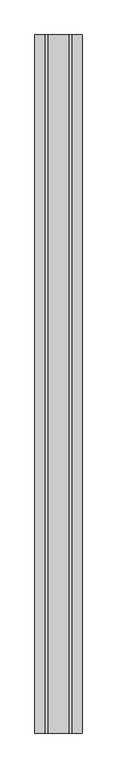
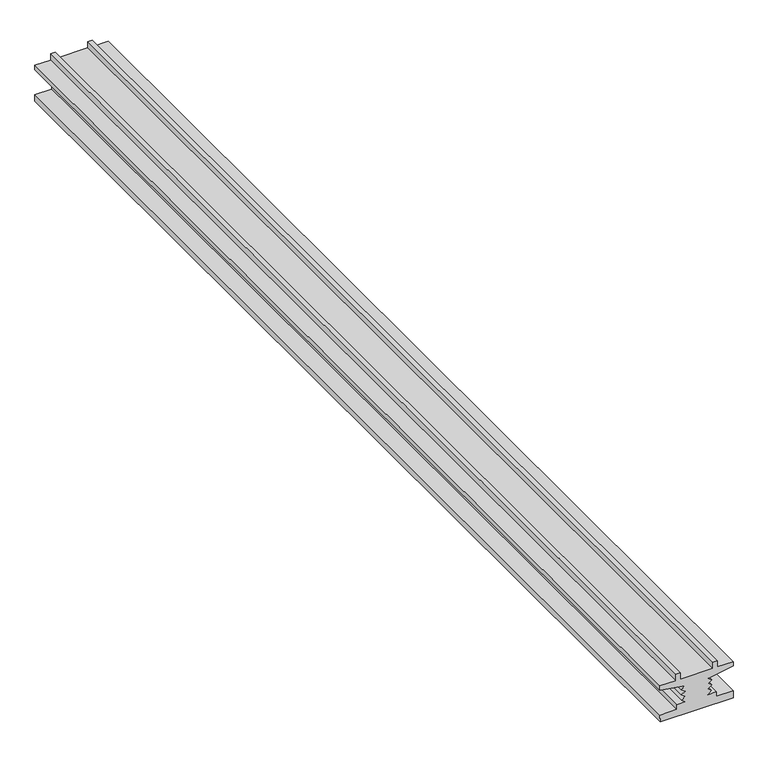
"""IFC4 building model written with IfcOpenShell, lengths in millimetres: proxy geometry, Bison pedestal001 : Bison pedestal001."""

import ifcopenshell
import ifcopenshell.guid

model = None  # the IFC model being written
_history = None  # IfcOwnerHistory: only IFC2X3 demands one
_inside = {}  # id of a spatial element -> (the spatial element, [elements in it])
_under = {}  # id of a project, library or spatial element -> (it, [spatial elements below it])
_declared = {}  # id of a project -> (the project, [libraries it declares])
_typed = {}  # id of a type object -> (the type object, [elements of that type])
_made_of = {}  # id of a material, layer set ... -> (it, [elements and type objects made of it])


def new_model(schema):
    """Start an empty IFC model of exactly this schema.

    Asked for "IFC4X3", IfcOpenShell would pick the latest addendum, in which some entities
    have other attributes; the version numbers below select the first issue.
    IFC2X3 requires an IfcOwnerHistory on every rooted entity: one is made here for all.
    """
    global model, _history
    if schema == "IFC4X3":
        model = ifcopenshell.file(schema_version=(4, 3, 0, 0))
    else:
        model = ifcopenshell.file(schema=schema)
    _inside.clear()
    _under.clear()
    _declared.clear()
    _typed.clear()
    _made_of.clear()
    _history = None
    if model.schema == "IFC2X3":
        org = make("IfcOrganization", Name="unknown")
        user = make(
            "IfcPersonAndOrganization",
            ThePerson=make("IfcPerson", FamilyName="unknown"),
            TheOrganization=org,
        )
        app = make(
            "IfcApplication",
            ApplicationDeveloper=org,
            Version="unknown",
            ApplicationFullName="unknown",
            ApplicationIdentifier="unknown",
        )
        _history = make(
            "IfcOwnerHistory",
            OwningUser=user,
            OwningApplication=app,
            ChangeAction="ADDED",
            CreationDate=0,
        )
    return model


def make(cls, **values):
    """One entity of the class cls with the attributes given. An attribute that is None is left unset."""
    return model.create_entity(
        cls, **{name: value for name, value in values.items() if value is not None}
    )


def rooted(cls, **values):
    """An entity with a GlobalId (a new one), such as an element, a storey or a relation."""
    return make(cls, GlobalId=ifcopenshell.guid.new(), OwnerHistory=_history, **values)


def si_unit(unit_type, name, prefix=None):
    """IfcSIUnit, for example si_unit("LENGTHUNIT", "METRE", prefix="MILLI")."""
    return make("IfcSIUnit", UnitType=unit_type, Prefix=prefix, Name=name)


def assignment(units):
    """IfcUnitAssignment: the units of a project."""
    return None if units is None else make("IfcUnitAssignment", Units=units)


def point(xyz):
    """IfcCartesianPoint."""
    return None if xyz is None else make("IfcCartesianPoint", Coordinates=xyz)


def direction(xyz):
    """IfcDirection."""
    return None if xyz is None else make("IfcDirection", DirectionRatios=xyz)


def frame(location, z_axis=None, x_axis=None):
    """IfcAxis2Placement3D, a coordinate frame: its origin and axes. An axis left out is left unset."""
    return make(
        "IfcAxis2Placement3D",
        Location=point(location),
        Axis=direction(z_axis),
        RefDirection=direction(x_axis),
    )


def origin():
    """The frame at (0, 0, 0) with its axes left unset."""
    return frame((0.0, 0.0, 0.0))


def place(relative_to, where):
    """IfcLocalPlacement: puts the frame where relative to a parent placement (None: the world)."""
    return make(
        "IfcLocalPlacement", PlacementRelTo=relative_to, RelativePlacement=where
    )


def context(
    kind, dimensions, precision=None, world=None, true_north=None, identifier=None
):
    """IfcGeometricRepresentationContext, for example the 3D "Model" context."""
    return make(
        "IfcGeometricRepresentationContext",
        ContextIdentifier=identifier,
        ContextType=kind,
        CoordinateSpaceDimension=dimensions,
        Precision=precision,
        WorldCoordinateSystem=world,
        TrueNorth=true_north,
    )


def project(units=None, contexts=None):
    """IfcProject with its units and contexts."""
    return rooted(
        "IfcProject",
        Name="project",
        RepresentationContexts=contexts,
        UnitsInContext=assignment(units),
    )


def spatial(cls, under=None, at=None, **own):
    """A site, building, storey or space (cls), placed at a placement, below another one or the project."""
    s = rooted(cls, ObjectPlacement=at, **own)
    if under is not None:
        _under.setdefault(under.id(), (under, []))[1].append(s)
    return s


def polyline(points):
    """IfcPolyline through the points."""
    return make("IfcPolyline", Points=[point(p) for p in points])


def outline(outer, holes=None, kind="AREA"):
    """IfcArbitraryClosedProfileDef: a profile drawn as a closed curve; with holes, ...WithVoids."""
    if holes is None:
        return make("IfcArbitraryClosedProfileDef", ProfileType=kind, OuterCurve=outer)
    return make(
        "IfcArbitraryProfileDefWithVoids",
        ProfileType=kind,
        OuterCurve=outer,
        InnerCurves=holes,
    )


def extrude(swept, where, along, depth):
    """IfcExtrudedAreaSolid: the profile swept, set in the frame where, extruded along a direction by depth."""
    return make(
        "IfcExtrudedAreaSolid",
        SweptArea=swept,
        Position=where,
        ExtrudedDirection=direction(along),
        Depth=depth,
    )


def shape(context_of_items, identifier, shape_type, items):
    """IfcShapeRepresentation: the items that make up one representation, for example the "Body"."""
    return make(
        "IfcShapeRepresentation",
        ContextOfItems=context_of_items,
        RepresentationIdentifier=identifier,
        RepresentationType=shape_type,
        Items=items,
    )


def source(mapping_origin, context_of_items, identifier, shape_type, items):
    """IfcRepresentationMap: a shape defined once, which mapped items show again and again."""
    return make(
        "IfcRepresentationMap",
        MappingOrigin=mapping_origin,
        MappedRepresentation=shape(context_of_items, identifier, shape_type, items),
    )


def transform(
    local_origin,
    x_axis=None,
    y_axis=None,
    z_axis=None,
    scale=None,
    scale2=None,
    scale3=None,
    uniform=True,
):
    """IfcCartesianTransformationOperator3D, or its non-uniform kind. x_axis, y_axis, z_axis: its Axis1, 2, 3."""
    if uniform:
        return make(
            "IfcCartesianTransformationOperator3D",
            Axis1=direction(x_axis),
            Axis2=direction(y_axis),
            LocalOrigin=point(local_origin),
            Scale=scale,
            Axis3=direction(z_axis),
        )
    return make(
        "IfcCartesianTransformationOperator3DnonUniform",
        Axis1=direction(x_axis),
        Axis2=direction(y_axis),
        LocalOrigin=point(local_origin),
        Scale=scale,
        Axis3=direction(z_axis),
        Scale2=scale2,
        Scale3=scale3,
    )


def mapped(mapping_source, mapping_target):
    """IfcMappedItem: shows the shape of a source again, moved by a transform."""
    return make(
        "IfcMappedItem", MappingSource=mapping_source, MappingTarget=mapping_target
    )


def made_of(thing, what):
    """Note that an element or type object is made of a material, layer set ...; save() writes the relation."""
    if what is not None:
        _made_of.setdefault(what.id(), (what, []))[1].append(thing)
    return thing


def element(
    cls,
    number,
    at=None,
    inside=None,
    cuts=None,
    type_object=None,
    material=None,
    context=None,
    identifier="Body",
    shape_type=None,
    held_by="IfcProductDefinitionShape",
    body=None,
    shapes=None,
    **own,
):
    """One element of the class cls, such as IfcWall. Its Tag is "e" and its number.

    at: its placement. inside: the storey or other place that contains it. cuts: it is an
    opening in that element (IfcRelVoidsElement). A single representation is given by context,
    identifier, shape_type and body (its items); several are given by shapes. held_by: the class
    of the entity that holds the representations. save() writes the other relations.
    """
    e = rooted(cls, Tag="e%d" % number, ObjectPlacement=at, **own)
    if body is not None:
        shapes = [shape(context, identifier, shape_type, body)]
    if shapes is not None:
        e.Representation = make(held_by, Representations=shapes)
    if inside is not None:
        _inside.setdefault(inside.id(), (inside, []))[1].append(e)
    if cuts is not None:
        rooted(
            "IfcRelVoidsElement", RelatingBuildingElement=cuts, RelatedOpeningElement=e
        )
    if type_object is not None:
        _typed.setdefault(type_object.id(), (type_object, []))[1].append(e)
    return made_of(e, material)


def aggregate(whole, parts):
    """IfcRelAggregates: a whole, such as a stair, and the parts it consists of."""
    return rooted("IfcRelAggregates", RelatingObject=whole, RelatedObjects=parts)


def save(model, path):
    """Write the relations noted so far, then the file.

    IfcRelAggregates (storeys below a building ...), IfcRelContainedInSpatialStructure (elements
    in a storey), IfcRelDefinesByType, IfcRelAssociatesMaterial and IfcRelDeclares: one each for
    every whole, place, type object, material and project.
    """
    for whole, parts in _under.values():
        aggregate(whole, parts)
    for where, things in _inside.values():
        rooted(
            "IfcRelContainedInSpatialStructure",
            RelatedElements=things,
            RelatingStructure=where,
        )
    for kind, things in _typed.values():
        rooted("IfcRelDefinesByType", RelatedObjects=things, RelatingType=kind)
    for what, things in _made_of.values():
        rooted("IfcRelAssociatesMaterial", RelatedObjects=things, RelatingMaterial=what)
    for by, libraries in _declared.values():
        rooted("IfcRelDeclares", RelatingContext=by, RelatedDefinitions=libraries)
    model.write(path)


def generic_models_6b344fbf(model_context):
    return source(origin(), model_context, "Body", "SweptSolid", [
        extrude(outline(polyline([(36449.6310479, -4803.6515856), (36463.03125, -4803.5224609), (36463.03125, -4834.3613281), (36471.986625, -4834.3613281), (36471.986625, -4850.543457), (36477.8694375, -4843.4819336), (36483.0217812, -4850.1020508), (36488.4631875, -4843.0410156), (36493.611625, -4849.8081055), (36498.6780312, -4842.6586914), (36503.7717812, -4849.0917969), (36511.5452187, -4803.5224609), (36519.8538125, -4803.5224609), (36519.8538125, -4833.0087891), (36532.1858437, -4833.0087891), (36532.1858437, -4840.7822266), (36519.8538125, -4840.7822266), (36519.8538125, -4901.3623047), (36532.1858437, -4901.3623047), (36532.1858437, -4909.1357422), (36519.8538125, -4909.1357422), (36519.8538125, -4938.6220703), (36511.5452187, -4938.6220703), (36503.7717812, -4893.0527344), (36498.6780312, -4899.4858398), (36493.611625, -4892.3364258), (36488.4631875, -4899.1035156), (36483.0217812, -4892.0424805), (36477.8694375, -4898.6625977), (36471.986625, -4891.6010742), (36471.986625, -4907.7832031), (36463.03125, -4907.7832031), (36463.03125, -4938.6220703), (36449.6310479, -4938.4929457), (36449.6310479, -4871.0722656), (36449.6310479, -4803.6515856)])), frame((0.0, -1052.8906574, 0.0), z_axis=(0.0, 1.0, 0.0), x_axis=(0.0, 0.0, 1.0)), (0.0, 0.0, 1.0), 2000.0),
    ])


if __name__ == "__main__":
    model = new_model("IFC4")
    model_context = context("Model", 3, world=origin())
    ifc_project = project(units=[si_unit("LENGTHUNIT", "METRE", prefix="MILLI")], contexts=[model_context])
    site = spatial("IfcSite", under=ifc_project)
    building = spatial("IfcBuilding", under=site)
    placement = place(None, origin())
    generic_models_shape = generic_models_6b344fbf(model_context)
    element("IfcBuildingElementProxy", 1, Name="Bison pedestal001 : Bison pedestal001", ObjectType="Bison pedestal001 : Bison pedestal001", at=placement, inside=building, context=model_context, shape_type="MappedRepresentation", body=[
        mapped(generic_models_shape, transform((0.0, 0.0, 0.0), x_axis=(1.0, 0.0, 0.0), y_axis=(0.0, 1.0, 0.0), z_axis=(0.0, 0.0, 1.0))),
    ])
    save(model, "model.ifc")

# Revit data of these elements
# Type "Bison pedestal001 : Bison pedestal001"
#   NameOverride = "Bison pedestal001"
# Element 1 (IfcBuildingElementProxy, "Bison pedestal001 : Bison pedestal001")
#   Materials on its faces: "BUZON PEDESTAL"
# Materials
#   "BUZON PEDESTAL": class "Unassigned", colour RGB 66 66 66, transparency 0
